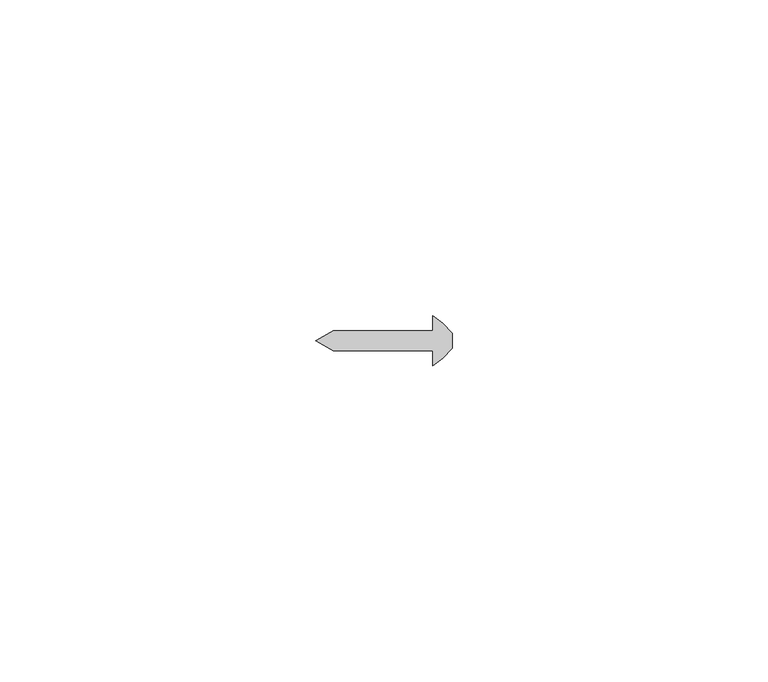
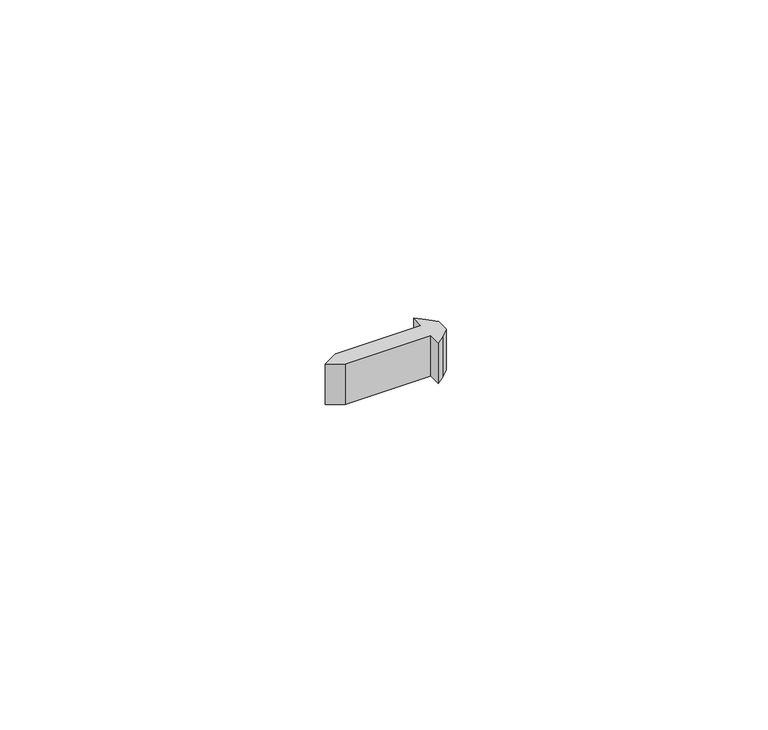
"""IFC4 building model written with IfcOpenShell, lengths in millimetres: proxy geometry, Generic Models 7:Generic Models 1:3:Generic Models 1:3 : Generic Models 7:Generic Models 1:305549:3:Generic Models 1:3:Generic Models 1:3 : Generic Models 7:Generic Models 1:305549:3 : Generic Models 7:Generic Models 1:3:Generic Models 1:3 : Generic Models 7:Generic Models 1:305549:301244:56 : Generic Models 7:Generic Models 1:3:Generic Models 1:3 : Generic Models 7:Generic Models 1:305549:3:Generic Models 1:3:Generic Models 1:3 : Generic Models 7:Generic Models 1:305549:3 : Generic Models 7:Generic Models 1:3:Generic Models 1:3 : Generic Models 7:Generic Models 1:305549:301244:308848."""

from ifc_helpers import new_model, si_unit, frame, origin, place, context, project, spatial, polyline, outline, extrude, source, transform, mapped, element, save


def generic_models_5ca85223(model_context):
    return source(origin(), model_context, "Body", "SweptSolid", [
        extrude(outline(polyline([(579391.8492239, -578751.4538841), (579376.0399684, -578751.4538841), (579373.2903377, -578749.8663841), (579376.0399684, -578748.2788841), (579391.8492239, -578748.2788841), (579391.8492239, -578745.8976341), (579393.3762819, -578747.1158297), (579394.9281721, -578748.6677199), (579394.9281721, -578751.0650483), (579393.3762819, -578752.6169385), (579391.8492239, -578753.8351341), (579391.8492239, -578751.4538841)])), frame((0.0, 0.0, 4907.75625), z_axis=(0.0, 0.0, 1.0), x_axis=(1.0, 0.0, 0.0)), (0.0, 0.0, 1.0), 7.9375),
    ])


if __name__ == "__main__":
    model = new_model("IFC4")
    model_context = context("Model", 3, world=origin())
    ifc_project = project(units=[si_unit("LENGTHUNIT", "METRE", prefix="MILLI")], contexts=[model_context])
    site = spatial("IfcSite", under=ifc_project)
    building = spatial("IfcBuilding", under=site)
    placement = place(None, origin())
    generic_models_shape = generic_models_5ca85223(model_context)
    element("IfcBuildingElementProxy", 1, Name="Generic Models 7:Generic Models 1:3:Generic Models 1:3 : Generic Models 7:Generic Models 1:305549:3:Generic Models 1:3:Generic Models 1:3 : Generic Models 7:Generic Models 1:305549:3 : Generic Models 7:Generic Models 1:3:Generic Models 1:3 : Generic Models 7:Generic Models 1:305549:301244:56 : Generic Models 7:Generic Models 1:3:Generic Models 1:3 : Generic Models 7:Generic Models 1:305549:3:Generic Models 1:3:Generic Models 1:3 : Generic Models 7:Generic Models 1:305549:3 : Generic Models 7:Generic Models 1:3:Generic Models 1:3 : Generic Models 7:Generic Models 1:305549:301244:308848", ObjectType="Generic Models 7:Generic Models 1:3:Generic Models 1:3 : Generic Models 7:Generic Models 1:305549:3:Generic Models 1:3:Generic Models 1:3 : Generic Models 7:Generic Models 1:305549:3 : Generic Models 7:Generic Models 1:3:Generic Models 1:3 : Generic Models 7:Generic Models 1:305549:301244:56 : Generic Models 7:Generic Models 1:3:Generic Models 1:3 : Generic Models 7:Generic Models 1:305549:3:Generic Models 1:3:Generic Models 1:3 : Generic Models 7:Generic Models 1:305549:3 : Generic Models 7:Generic Models 1:3:Generic Models 1:3 : Generic Models 7:Generic Models 1:305549:301244:308848", at=placement, inside=building, context=model_context, shape_type="MappedRepresentation", body=[
        mapped(generic_models_shape, transform((0.0, 0.0, 0.0), x_axis=(1.0, 0.0, 0.0), y_axis=(0.0, 1.0, 0.0), z_axis=(0.0, 0.0, 1.0))),
    ])
    save(model, "model.ifc")

# Revit data of these elements
# Type "Generic Models 7:Generic Models 1:3:Generic Models 1:3 : Generic Models 7:Generic Models 1:305549:3:Generic Models 1:3:Generic Models 1:3 : Generic Models 7:Generic Models 1:305549:3 : Generic Models 7:Generic Models 1:3:Generic Models 1:3 : Generic Models 7:Generic Models 1:305549:301244:56 : Generic Models 7:Generic Models 1:3:Generic Models 1:3 : Generic Models 7:Generic Models 1:305549:3:Generic Models 1:3:Generic Models 1:3 : Generic Models 7:Generic Models 1:305549:3 : Generic Models 7:Generic Models 1:3:Generic Models 1:3 : Generic Models 7:Generic Models 1:305549:301244:308848"
#   NameOverride = "Generic Models 7:Generic Models 1:3:Generic Models 1:3 : Generic Models 7:Generic Models 1:305549:3:Generic Models 1:3:Generic Models 1:3 : Generic Models 7:Generic Models 1:305549:3 : Generic Models 7:Generic Models 1:3:Generic Models 1:3 : Generic Models 7:Generic Models 1:305549:301244:308848"
#   ObjectTypeOverride = "Generic Models 1:3:Generic Models 1:3 : Generic Models 7:Generic Models 1:305549:3 : Generic Models 7:Generic Models 1:3:Generic Models 1:3 : Generic Models 7:Generic Models 1:305549:301244"
#   Reference = "Generic Models 1"
#   Tag = "308848"
# Element 1 (IfcBuildingElementProxy, "Generic Models 7:Generic Models 1:3:Generic Models 1:3 : Generic Models 7:Generic Models 1:305549:3:Generic Models 1:3:Generic Models 1:3 : Generic Models 7:Generic Models 1:305549:3 : Generic Models 7:Generic Models 1:3:Generic Models 1:3 : Generic Models 7:Generic Models 1:305549:301244:56 : Generic Models 7:Generic Models 1:3:Generic Models 1:3 : Generic Models 7:Generic Models 1:305549:3:Generic Models 1:3:Generic Models 1:3 : Generic Models 7:Generic Models 1:305549:3 : Generic Models 7:Generic Models 1:3:Generic Models 1:3 : Generic Models 7:Generic Models 1:305549:301244:308848")
#   Materials on its faces: "FASTENERS (T.B.D)"
# Materials
#   "FASTENERS (T.B.D)": class "Generic", colour RGB 120 120 120, transparency 0, Cost = 0
